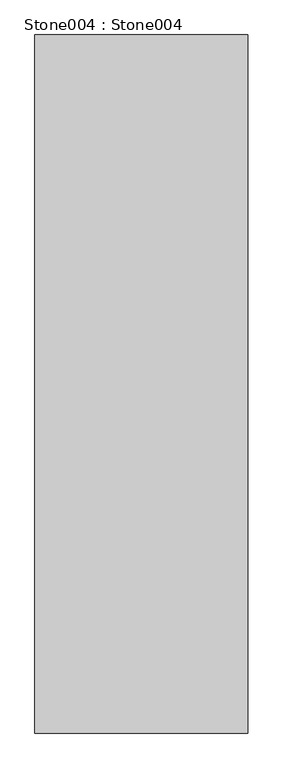
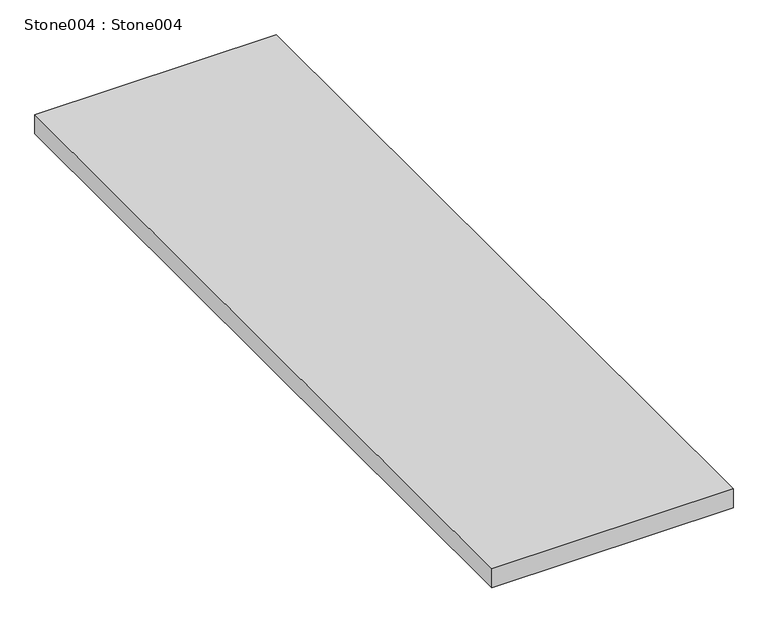
"""IFC4 building model written with IfcOpenShell, lengths in millimetres: proxy geometry, Stone004 : Stone004."""

from ifc_helpers import new_model, si_unit, frame, origin, place, context, project, spatial, polyline, outline, extrude, source, transform, mapped, element, save


def stone004_stone004_df4a59c1(model_context):
    return source(origin(), model_context, "Body", "SweptSolid", [
        extrude(outline(polyline([(-3623.2530392, -1052.8906574), (-4232.8530392, -1052.8906574), (-4232.8530392, 947.1093426), (-3623.2530392, 947.1093426), (-3623.2530392, -1052.8906574)])), frame((0.0, 0.0, 36518.596), z_axis=(0.0, 0.0, 1.0), x_axis=(1.0, 0.0, 0.0)), (0.0, 0.0, 1.0), 50.8),
    ])


if __name__ == "__main__":
    model = new_model("IFC4")
    model_context = context("Model", 3, world=origin())
    ifc_project = project(units=[si_unit("LENGTHUNIT", "METRE", prefix="MILLI")], contexts=[model_context])
    site = spatial("IfcSite", under=ifc_project)
    building = spatial("IfcBuilding", under=site)
    placement = place(None, origin())
    stone004_stone004_shape = stone004_stone004_df4a59c1(model_context)
    element("IfcBuildingElementProxy", 1, Name="Stone004 : Stone004", ObjectType="Stone004 : Stone004", at=placement, inside=building, context=model_context, shape_type="MappedRepresentation", body=[
        mapped(stone004_stone004_shape, transform((0.0, 0.0, 0.0), x_axis=(1.0, 0.0, 0.0), y_axis=(0.0, 1.0, 0.0), z_axis=(0.0, 0.0, 1.0))),
    ])
    save(model, "model.ifc")

# Revit data of these elements
# Type "Stone004 : Stone004"
#   NameOverride = "Stone004"
# Element 1 (IfcBuildingElementProxy, "Stone004 : Stone004")
#   Materials on its faces: "2\" STONE DECK TBD"
# Materials
#   "2\" STONE DECK TBD": class "Unassigned", colour RGB 199 185 173, transparency 0
